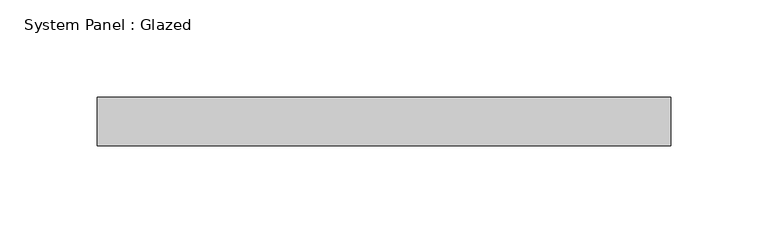
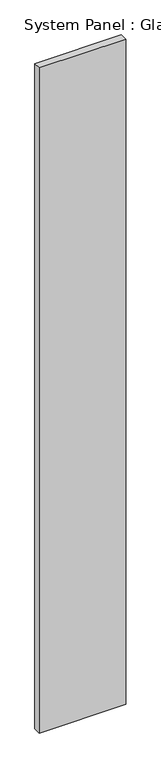
"""IFC4 building model written with IfcOpenShell, lengths in millimetres: plate geometry, System Panel : Glazed."""

from ifc_helpers import new_model, si_unit, origin, origin_with_axes, place, context, project, spatial, polyline, outline, extrude, source, transform, mapped, element, save


def system_panel_glazed_f7563303(model_context):
    return source(origin(), model_context, "Body", "SweptSolid", [
        extrude(outline(polyline([(147.4999998, 24.5), (-147.4999998, 24.5), (-147.4999998, 49.5), (147.4999998, 49.5), (147.4999998, 24.5)])), origin_with_axes(), (0.0, 0.0, 1.0), 2400.0),
    ])


if __name__ == "__main__":
    model = new_model("IFC4")
    model_context = context("Model", 3, world=origin())
    ifc_project = project(units=[si_unit("LENGTHUNIT", "METRE", prefix="MILLI")], contexts=[model_context])
    site = spatial("IfcSite", under=ifc_project)
    building = spatial("IfcBuilding", under=site)
    placement = place(None, origin())
    system_panel_glazed_shape = system_panel_glazed_f7563303(model_context)
    element("IfcPlate", 1, ObjectType="System Panel : Glazed", at=placement, inside=building, context=model_context, shape_type="MappedRepresentation", body=[
        mapped(system_panel_glazed_shape, transform((0.0, 0.0, 0.0), x_axis=(1.0, 0.0, 0.0), y_axis=(0.0, 1.0, 0.0), z_axis=(0.0, 0.0, 1.0))),
    ])
    save(model, "model.ifc")

# Revit data of these elements
# Type "System Panel : Glazed"
#   Keynote = "H11"
#   Construction Type Id = "GSP4R"
#   Analytic Construction = "1/8 in Pilkington single glazing"
#   Visual Light Transmittance = 0.9
#   Solar Heat Gain Coefficient = 0.86
#   Heat Transfer Coefficient (U) = 6.7069 W/(m²·K)
#   Define Thermal Properties by = 1
# Element 1 (IfcPlate, "System Panel : Glazed")
#   Materials on its faces: "Glass"
# Materials
#   "Glass": class "Glass", colour RGB 0 128 192, transparency 0.9, Description = "Soda Lime Glass", Cost = 0
